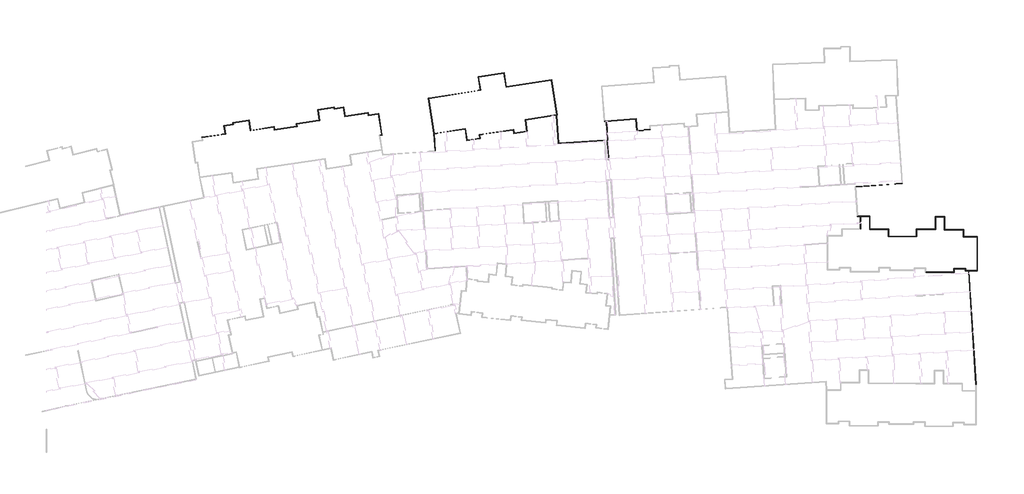
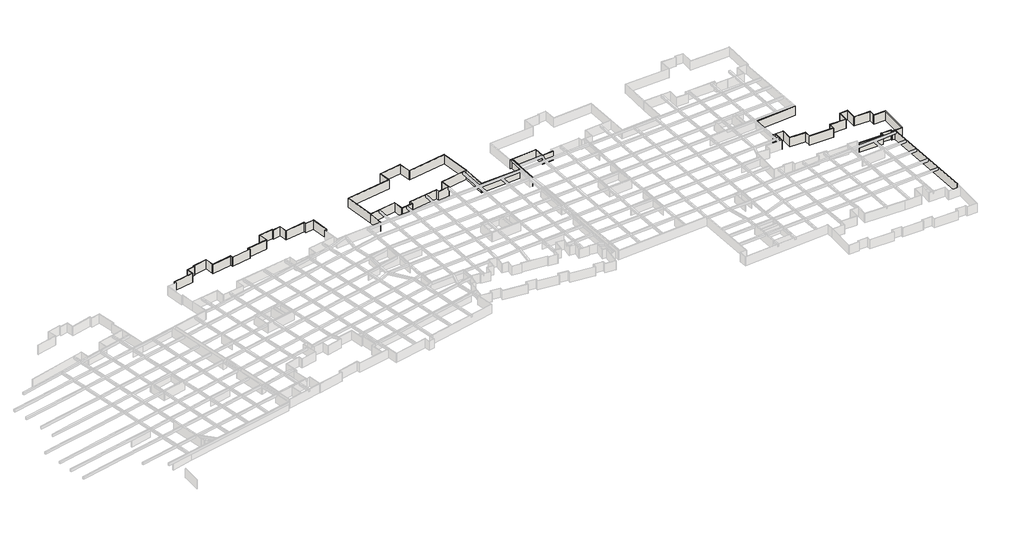
# One storey, part 6 of 14: 66 walls.
"""IFC4 building model written with IfcOpenShell, lengths in millimetres."""

from ifc_helpers import new_model, si_unit, origin, origin_with_axes, place, context, project, spatial, polyline, outline, extrude, faceted_brep, element, save

model = new_model("IFC4")

# Units and contexts
model_context = context("Model", 3, world=origin())
ifc_project = project(units=[si_unit("LENGTHUNIT", "METRE", prefix="MILLI")], contexts=[model_context])

# Site, building, storey
site = spatial("IfcSite", under=ifc_project)
building = spatial("IfcBuilding", under=site)
storey = spatial("IfcBuildingStorey", under=building, Name="户型图", Elevation=0.0)

# Walls
placement = place(None, origin())
element("IfcWall", 1, ObjectType="所有墙体", at=placement, inside=storey, context=model_context, shape_type="Brep", body=[
    faceted_brep([(-63852.357784, -149438.6682209, 0.0), (-63852.357784, -153118.7611434, 0.0), (-63852.357784, -153238.7611434, 0.0), (-63852.357784, -153238.7611434, 3300.0), (-63852.357784, -153118.7611434, 3300.0), (-63852.357784, -149438.6682209, 3300.0), (-63732.357784, -149438.6682209, 0.0), (-63732.357784, -149438.6682209, 3300.0), (-63732.357784, -153238.7611434, 3300.0), (-63732.357784, -153238.7611434, 0.0)], [[[0, 1, 2, 3, 4, 5]], [[6, 7, 8, 9]], [[2, 1, 0, 6, 9]], [[5, 4, 3, 8, 7]], [[3, 2, 9, 8]], [[0, 5, 7, 6]]]),
])
element("IfcWall", 2, ObjectType="所有墙体", at=placement, inside=storey, context=model_context, shape_type="Brep", body=[
    faceted_brep([(-44489.8483382, -166077.0504792, 0.0), (-36098.0374087, -166077.0504792, 0.0), (-36098.0374087, -166077.0504792, 3300.0), (-44489.8483382, -166077.0504792, 3300.0), (-44489.8483382, -165957.0504792, 0.0), (-44489.8483382, -165957.0504792, 3300.0), (-36218.0374087, -165957.0504792, 3300.0), (-36098.0374087, -165957.0504792, 3300.0), (-36098.0374087, -165957.0504792, 0.0), (-36218.0374087, -165957.0504792, 0.0)], [[[0, 1, 2, 3]], [[4, 5, 6, 7, 8, 9]], [[1, 0, 4, 9, 8]], [[3, 2, 7, 6, 5]], [[0, 3, 5, 4]], [[2, 1, 8, 7]]]),
])
element("IfcWall", 3, ObjectType="所有墙体", at=placement, inside=storey, context=model_context, shape_type="Brep", body=[
    faceted_brep([(-36098.0374087, -165957.0504792, 0.0), (-36098.0374087, -165032.3015604, 0.0), (-36098.0374087, -164912.3015604, 0.0), (-36098.0374087, -164817.0504792, 0.0), (-36098.0374087, -164817.0504792, 3300.0), (-36098.0374087, -164912.3015604, 3300.0), (-36098.0374087, -165032.3015604, 3300.0), (-36098.0374087, -165957.0504792, 3300.0), (-36218.0374087, -165957.0504792, 0.0), (-36218.0374087, -165957.0504792, 3300.0), (-36218.0374087, -164817.0504792, 3300.0), (-36218.0374087, -164817.0504792, 0.0)], [[[0, 1, 2, 3, 4, 5, 6, 7]], [[8, 9, 10, 11]], [[3, 2, 1, 0, 8, 11]], [[4, 3, 11, 10]], [[7, 6, 5, 4, 10, 9]], [[0, 7, 9, 8]]]),
])
element("IfcWall", 4, ObjectType="所有墙体", at=placement, inside=storey, context=model_context, shape_type="Brep", body=[
    faceted_brep([(-36098.0374087, -165032.3015604, 0.0), (-32810.647962, -165032.3015604, 0.0), (-32690.647962, -165032.3015604, 0.0), (-32690.647962, -165032.3015604, 3300.0), (-32810.647962, -165032.3015604, 3300.0), (-36098.0374087, -165032.3015604, 3300.0), (-36098.0374087, -164912.3015604, 0.0), (-36098.0374087, -164912.3015604, 3300.0), (-32690.647962, -164912.3015604, 3300.0), (-32690.647962, -164912.3015604, 0.0)], [[[0, 1, 2, 3, 4, 5]], [[6, 7, 8, 9]], [[2, 1, 0, 6, 9]], [[5, 4, 3, 8, 7]], [[0, 5, 7, 6]], [[3, 2, 9, 8]]]),
])
element("IfcWall", 5, ObjectType="所有墙体", at=placement, inside=storey, context=model_context, shape_type="Brep", body=[
    faceted_brep([(-32810.647962, -165032.3015604, 0.0), (-32810.647962, -165556.1428891, 0.0), (-32810.647962, -165556.1428891, 3300.0), (-32810.647962, -165032.3015604, 3300.0), (-32690.647962, -165032.3015604, 0.0), (-32690.647962, -165032.3015604, 3300.0), (-32690.647962, -165436.1428891, 3300.0), (-32690.647962, -165556.1428891, 3300.0), (-32690.647962, -165556.1428891, 0.0), (-32690.647962, -165436.1428891, 0.0)], [[[0, 1, 2, 3]], [[4, 5, 6, 7, 8, 9]], [[1, 0, 4, 9, 8]], [[3, 2, 7, 6, 5]], [[0, 3, 5, 4]], [[2, 1, 8, 7]]]),
])
element("IfcWall", 6, ObjectType="所有墙体", at=placement, inside=storey, context=model_context, shape_type="Brep", body=[
    faceted_brep([(-32690.647962, -165556.1428891, 0.0), (-31833.0771773, -165556.1428891, 0.0), (-31712.8241848, -165556.1428891, 0.0), (-29194.2257868, -165556.1428891, 0.0), (-29194.2257868, -165556.1428891, 3300.0), (-31712.8241848, -165556.1428891, 3300.0), (-31833.0771773, -165556.1428891, 3300.0), (-32690.647962, -165556.1428891, 3300.0), (-32690.647962, -165436.1428891, 0.0), (-32690.647962, -165436.1428891, 3300.0), (-29314.2257868, -165436.1428891, 3300.0), (-29194.2257868, -165436.1428891, 3300.0), (-29194.2257868, -165436.1428891, 0.0), (-29314.2257868, -165436.1428891, 0.0)], [[[0, 1, 2, 3, 4, 5, 6, 7]], [[8, 9, 10, 11, 12, 13]], [[3, 2, 1, 0, 8, 13, 12]], [[7, 6, 5, 4, 11, 10, 9]], [[0, 7, 9, 8]], [[4, 3, 12, 11]]]),
])
element("IfcWall", 7, ObjectType="所有墙体", at=placement, inside=storey, context=model_context, shape_type="Brep", body=[
    faceted_brep([(-29194.2257868, -165436.1428891, 0.0), (-29194.2257868, -155436.1428891, 0.0), (-29194.2257868, -155436.1428891, 3300.0), (-29194.2257868, -165436.1428891, 3300.0), (-29314.2257868, -165436.1428891, 0.0), (-29314.2257868, -165436.1428891, 3300.0), (-29314.2257868, -155556.1428891, 3300.0), (-29314.2257868, -155436.1428891, 3300.0), (-29314.2257868, -155436.1428891, 0.0), (-29314.2257868, -155556.1428891, 0.0)], [[[0, 1, 2, 3]], [[4, 5, 6, 7, 8, 9]], [[1, 0, 4, 9, 8]], [[3, 2, 7, 6, 5]], [[0, 3, 5, 4]], [[2, 1, 8, 7]]]),
])
element("IfcWall", 8, ObjectType="所有墙体", at=placement, inside=storey, context=model_context, shape_type="Brep", body=[
    faceted_brep([(-29314.2257868, -155436.1428891, 0.0), (-33294.2257868, -155436.1428891, 0.0), (-33414.2257868, -155436.1428891, 0.0), (-33414.2257868, -155436.1428891, 3300.0), (-33294.2257868, -155436.1428891, 3300.0), (-29314.2257868, -155436.1428891, 3300.0), (-29314.2257868, -155556.1428891, 0.0), (-29314.2257868, -155556.1428891, 3300.0), (-33414.2257868, -155556.1428891, 3300.0), (-33414.2257868, -155556.1428891, 0.0)], [[[0, 1, 2, 3, 4, 5]], [[6, 7, 8, 9]], [[2, 1, 0, 6, 9]], [[5, 4, 3, 8, 7]], [[0, 5, 7, 6]], [[3, 2, 9, 8]]]),
])
element("IfcWall", 9, ObjectType="所有墙体", at=placement, inside=storey, context=model_context, shape_type="Brep", body=[
    faceted_brep([(-33294.2257868, -155436.1428891, 0.0), (-33294.2257868, -153331.6259677, 0.0), (-33294.2257868, -153331.6259677, 3300.0), (-33294.2257868, -155436.1428891, 3300.0), (-33414.2257868, -155436.1428891, 0.0), (-33414.2257868, -155436.1428891, 3300.0), (-33414.2257868, -153451.6259677, 3300.0), (-33414.2257868, -153331.6259677, 3300.0), (-33414.2257868, -153331.6259677, 0.0), (-33414.2257868, -153451.6259677, 0.0)], [[[0, 1, 2, 3]], [[4, 5, 6, 7, 8, 9]], [[1, 0, 4, 9, 8]], [[3, 2, 7, 6, 5]], [[0, 3, 5, 4]], [[2, 1, 8, 7]]]),
])
element("IfcWall", 10, ObjectType="所有墙体", at=placement, inside=storey, context=model_context, shape_type="Brep", body=[
    faceted_brep([(-33414.2257868, -153331.6259677, 0.0), (-38859.8129577, -153331.6259677, 0.0), (-38979.8129577, -153331.6259677, 0.0), (-38979.8129577, -153331.6259677, 3300.0), (-38859.8129577, -153331.6259677, 3300.0), (-33414.2257868, -153331.6259677, 3300.0), (-33414.2257868, -153451.6259677, 0.0), (-33414.2257868, -153451.6259677, 3300.0), (-38979.8129577, -153451.6259677, 3300.0), (-38979.8129577, -153451.6259677, 0.0)], [[[0, 1, 2, 3, 4, 5]], [[6, 7, 8, 9]], [[2, 1, 0, 6, 9]], [[5, 4, 3, 8, 7]], [[0, 5, 7, 6]], [[3, 2, 9, 8]]]),
])
element("IfcWall", 11, ObjectType="所有墙体", at=placement, inside=storey, context=model_context, shape_type="Brep", body=[
    faceted_brep([(-38859.8129577, -153331.6259677, 0.0), (-38859.8129577, -149531.6259677, 0.0), (-38859.8129577, -149531.6259677, 3300.0), (-38859.8129577, -153331.6259677, 3300.0), (-38979.8129577, -153331.6259677, 0.0), (-38979.8129577, -153331.6259677, 3300.0), (-38979.8129577, -149651.6259677, 3300.0), (-38979.8129577, -149531.6259677, 3300.0), (-38979.8129577, -149531.6259677, 0.0), (-38979.8129577, -149651.6259677, 0.0)], [[[0, 1, 2, 3]], [[4, 5, 6, 7, 8, 9]], [[1, 0, 4, 9, 8]], [[3, 2, 7, 6, 5]], [[0, 3, 5, 4]], [[2, 1, 8, 7]]]),
])
element("IfcWall", 12, ObjectType="所有墙体", at=placement, inside=storey, context=model_context, shape_type="Brep", body=[
    faceted_brep([(-38979.8129577, -149531.6259677, 0.0), (-41679.8129577, -149531.6259677, 0.0), (-41679.8129577, -149531.6259677, 3300.0), (-38979.8129577, -149531.6259677, 3300.0), (-38979.8129577, -149651.6259677, 0.0), (-38979.8129577, -149651.6259677, 3300.0), (-41559.8129577, -149651.6259677, 3300.0), (-41679.8129577, -149651.6259677, 3300.0), (-41679.8129577, -149651.6259677, 0.0), (-41559.8129577, -149651.6259677, 0.0)], [[[0, 1, 2, 3]], [[4, 5, 6, 7, 8, 9]], [[1, 0, 4, 9, 8]], [[3, 2, 7, 6, 5]], [[0, 3, 5, 4]], [[2, 1, 8, 7]]]),
])
element("IfcWall", 13, ObjectType="所有墙体", at=placement, inside=storey, context=model_context, shape_type="Brep", body=[
    faceted_brep([(-41679.8129577, -149651.6259677, 0.0), (-41679.8129577, -153231.6259677, 0.0), (-41679.8129577, -153351.6259677, 0.0), (-41679.8129577, -153351.6259677, 3300.0), (-41679.8129577, -153231.6259677, 3300.0), (-41679.8129577, -149651.6259677, 3300.0), (-41559.8129577, -149651.6259677, 0.0), (-41559.8129577, -149651.6259677, 3300.0), (-41559.8129577, -153351.6259677, 3300.0), (-41559.8129577, -153351.6259677, 0.0)], [[[0, 1, 2, 3, 4, 5]], [[6, 7, 8, 9]], [[2, 1, 0, 6, 9]], [[5, 4, 3, 8, 7]], [[0, 5, 7, 6]], [[3, 2, 9, 8]]]),
])
element("IfcWall", 14, ObjectType="所有墙体", at=placement, inside=storey, context=model_context, shape_type="Brep", body=[
    faceted_brep([(-41679.8129577, -153231.6259677, 0.0), (-47279.8129577, -153231.6259677, 0.0), (-47279.8129577, -153231.6259677, 3300.0), (-41679.8129577, -153231.6259677, 3300.0), (-41679.8129577, -153351.6259677, 0.0), (-41679.8129577, -153351.6259677, 3300.0), (-47159.8129577, -153351.6259677, 3300.0), (-47279.8129577, -153351.6259677, 3300.0), (-47279.8129577, -153351.6259677, 0.0), (-47159.8129577, -153351.6259677, 0.0)], [[[0, 1, 2, 3]], [[4, 5, 6, 7, 8, 9]], [[1, 0, 4, 9, 8]], [[3, 2, 7, 6, 5]], [[0, 3, 5, 4]], [[2, 1, 8, 7]]]),
])
element("IfcWall", 15, ObjectType="所有墙体", at=placement, inside=storey, context=model_context, shape_type="Brep", body=[
    faceted_brep([(-47279.8129577, -153351.6259677, 0.0), (-47279.8129577, -155331.6259677, 0.0), (-47279.8129577, -155451.6259677, 0.0), (-47279.8129577, -155451.6259677, 3300.0), (-47279.8129577, -155331.6259677, 3300.0), (-47279.8129577, -153351.6259677, 3300.0), (-47159.8129577, -153351.6259677, 0.0), (-47159.8129577, -153351.6259677, 3300.0), (-47159.8129577, -155451.6259677, 3300.0), (-47159.8129577, -155451.6259677, 0.0)], [[[0, 1, 2, 3, 4, 5]], [[6, 7, 8, 9]], [[2, 1, 0, 6, 9]], [[5, 4, 3, 8, 7]], [[0, 5, 7, 6]], [[3, 2, 9, 8]]]),
])
element("IfcWall", 16, ObjectType="所有墙体", at=placement, inside=storey, context=model_context, shape_type="Brep", body=[
    faceted_brep([(-47279.8129577, -155331.6259677, 0.0), (-55524.2068249, -155331.6259677, 0.0), (-55644.2068249, -155331.6259677, 0.0), (-55644.2068249, -155331.6259677, 3300.0), (-55524.2068249, -155331.6259677, 3300.0), (-47279.8129577, -155331.6259677, 3300.0), (-47279.8129577, -155451.6259677, 0.0), (-47279.8129577, -155451.6259677, 3300.0), (-55644.2068249, -155451.6259677, 3300.0), (-55644.2068249, -155451.6259677, 0.0)], [[[0, 1, 2, 3, 4, 5]], [[6, 7, 8, 9]], [[2, 1, 0, 6, 9]], [[5, 4, 3, 8, 7]], [[0, 5, 7, 6]], [[3, 2, 9, 8]]]),
])
element("IfcWall", 17, ObjectType="所有墙体", at=placement, inside=storey, context=model_context, shape_type="Brep", body=[
    faceted_brep([(-55524.2068249, -155331.6259677, 0.0), (-55524.2068249, -153151.6259677, 0.0), (-55524.2068249, -153151.6259677, 3300.0), (-55524.2068249, -155331.6259677, 3300.0), (-55644.2068249, -155331.6259677, 0.0), (-55644.2068249, -155331.6259677, 3300.0), (-55644.2068249, -153271.6259677, 3300.0), (-55644.2068249, -153151.6259677, 3300.0), (-55644.2068249, -153151.6259677, 0.0), (-55644.2068249, -153271.6259677, 0.0)], [[[0, 1, 2, 3]], [[4, 5, 6, 7, 8, 9]], [[1, 0, 4, 9, 8]], [[3, 2, 7, 6, 5]], [[0, 3, 5, 4]], [[2, 1, 8, 7]]]),
])
element("IfcWall", 18, ObjectType="所有墙体", at=placement, inside=storey, context=model_context, shape_type="Brep", body=[
    faceted_brep([(-55644.2068249, -153151.6259677, 0.0), (-61024.2068249, -153151.6259677, 0.0), (-61144.2068249, -153151.6259677, 0.0), (-61144.2068249, -153151.6259677, 3300.0), (-61024.2068249, -153151.6259677, 3300.0), (-55644.2068249, -153151.6259677, 3300.0), (-55644.2068249, -153271.6259677, 0.0), (-55644.2068249, -153271.6259677, 3300.0), (-61144.2068249, -153271.6259677, 3300.0), (-61144.2068249, -153271.6259677, 0.0)], [[[0, 1, 2, 3, 4, 5]], [[6, 7, 8, 9]], [[2, 1, 0, 6, 9]], [[5, 4, 3, 8, 7]], [[0, 5, 7, 6]], [[3, 2, 9, 8]]]),
])
element("IfcWall", 19, ObjectType="所有墙体", at=placement, inside=storey, context=model_context, shape_type="Brep", body=[
    faceted_brep([(-61024.2068249, -153151.6259677, 0.0), (-61024.2068249, -149318.6682209, 0.0), (-61024.2068249, -149318.6682209, 3300.0), (-61024.2068249, -153151.6259677, 3300.0), (-61144.2068249, -153151.6259677, 0.0), (-61144.2068249, -153151.6259677, 3300.0), (-61144.2068249, -149438.6682209, 3300.0), (-61144.2068249, -149318.6682209, 3300.0), (-61144.2068249, -149318.6682209, 0.0), (-61144.2068249, -149438.6682209, 0.0)], [[[0, 1, 2, 3]], [[4, 5, 6, 7, 8, 9]], [[1, 0, 4, 9, 8]], [[3, 2, 7, 6, 5]], [[0, 3, 5, 4]], [[2, 1, 8, 7]]]),
])
element("IfcWall", 20, ObjectType="所有墙体", at=placement, inside=storey, context=model_context, shape_type="Brep", body=[
    faceted_brep([(-61144.2068249, -149318.6682209, 0.0), (-64662.1102247, -149318.6682209, 0.0), (-64782.4032525, -149318.6682209, 0.0), (-64782.4032525, -149318.6682209, 3300.0), (-64662.1102247, -149318.6682209, 3300.0), (-61144.2068249, -149318.6682209, 3300.0), (-61144.2068249, -149438.6682209, 0.0), (-61144.2068249, -149438.6682209, 3300.0), (-63732.357784, -149438.6682209, 3300.0), (-63852.357784, -149438.6682209, 3300.0), (-64774.0120351, -149438.6682209, 3300.0), (-64774.0120351, -149438.6682209, 0.0), (-63852.357784, -149438.6682209, 0.0), (-63732.357784, -149438.6682209, 0.0)], [[[0, 1, 2, 3, 4, 5]], [[6, 7, 8, 9, 10, 11, 12, 13]], [[2, 1, 0, 6, 13, 12, 11]], [[5, 4, 3, 10, 9, 8, 7]], [[0, 5, 7, 6]], [[3, 2, 11, 10]]]),
])
element("IfcWall", 21, ObjectType="所有墙体", at=placement, inside=storey, context=model_context, shape_type="Brep", body=[
    faceted_brep([(-139619.0065176, -121289.1155096, 0.0), (-139081.9141821, -121248.6544174, 0.0), (-138962.222053, -121239.63758, 0.0), (-130362.6959186, -120591.8044292, 0.0), (-130243.034985, -120582.7899419, 0.0), (-130243.034985, -120582.7899419, 3300.0), (-130362.6959186, -120591.8044292, 3300.0), (-138962.222053, -121239.63758, 3300.0), (-139081.9141821, -121248.6544174, 3300.0), (-139619.0065176, -121289.1155096, 3300.0), (-139628.021005, -121169.4545761, 0.0), (-139628.021005, -121169.4545761, 3300.0), (-130252.0494724, -120463.1290083, 3300.0), (-130252.0494724, -120463.1290083, 0.0)], [[[0, 1, 2, 3, 4, 5, 6, 7, 8, 9]], [[10, 11, 12, 13]], [[4, 3, 2, 1, 0, 10, 13]], [[9, 8, 7, 6, 5, 12, 11]], [[0, 9, 11, 10]], [[5, 4, 13, 12]]]),
])
element("IfcWall", 22, ObjectType="所有墙体", at=placement, inside=storey, context=model_context, shape_type="Brep", body=[
    faceted_brep([(-130362.6959186, -120591.8044292, 0.0), (-130099.9459312, -124079.6243728, 0.0), (-130099.9459312, -124079.6243728, 3300.0), (-130362.6959186, -120591.8044292, 3300.0), (-130243.034985, -120582.7899419, 0.0), (-130243.034985, -120582.7899419, 3300.0), (-129989.299485, -123950.9489519, 3300.0), (-129980.2849976, -124070.6098855, 3300.0), (-129980.2849976, -124070.6098855, 0.0), (-129989.299485, -123950.9489519, 0.0)], [[[0, 1, 2, 3]], [[4, 5, 6, 7, 8, 9]], [[1, 0, 4, 9, 8]], [[3, 2, 7, 6, 5]], [[0, 3, 5, 4]], [[2, 1, 8, 7]]]),
])
element("IfcWall", 23, ObjectType="所有墙体", at=placement, inside=storey, context=model_context, shape_type="Brep", body=[
    faceted_brep([(-129980.2849976, -124070.6098855, 0.0), (-126090.4525069, -123777.5748509, 0.0), (-126090.4525069, -123777.5748509, 3300.0), (-129980.2849976, -124070.6098855, 3300.0), (-129989.299485, -123950.9489519, 0.0), (-129989.299485, -123950.9489519, 3300.0), (-126219.1279278, -123666.9284047, 3300.0), (-126099.4669943, -123657.9139173, 3300.0), (-126099.4669943, -123657.9139173, 0.0), (-126219.1279278, -123666.9284047, 0.0)], [[[0, 1, 2, 3]], [[4, 5, 6, 7, 8, 9]], [[1, 0, 4, 9, 8]], [[3, 2, 7, 6, 5]], [[0, 3, 5, 4]], [[2, 1, 8, 7]]]),
])
element("IfcWall", 24, ObjectType="所有墙体", at=placement, inside=storey, context=model_context, shape_type="Brep", body=[
    faceted_brep([(-190088.7056475, -124948.17441, 0.0), (-190107.4777833, -124829.6518091, 0.0), (-191744.4589692, -114494.1593671, 0.0), (-191763.231105, -114375.6367662, 0.0), (-191763.231105, -114375.6367662, 3300.0), (-191744.4589692, -114494.1593671, 3300.0), (-190107.4777833, -124829.6518091, 3300.0), (-190088.7056475, -124948.17441, 3300.0), (-190207.2282484, -124966.9465458, 0.0), (-190207.2282484, -124966.9465458, 3300.0), (-191881.7537059, -114394.408902, 3300.0), (-191881.7537059, -114394.408902, 0.0), (-190093.6639709, -124948.9597313, 0.0), (-190093.6639709, -124948.9597313, 3300.0)], [[[0, 1, 2, 3, 4, 5, 6, 7]], [[8, 9, 10, 11]], [[3, 2, 1, 0, 12, 8, 11]], [[7, 6, 5, 4, 10, 9, 13]], [[4, 3, 11, 10]], [[0, 7, 13, 9, 8, 12]]]),
])
element("IfcWall", 25, ObjectType="所有墙体", at=placement, inside=storey, context=model_context, shape_type="Brep", body=[
    faceted_brep([(-191744.4589692, -114494.1593671, 0.0), (-176350.1815066, -112055.945347, 0.0), (-176350.1815066, -112055.945347, 3300.0), (-191744.4589692, -114494.1593671, 3300.0), (-191763.231105, -114375.6367662, 0.0), (-191763.231105, -114375.6367662, 3300.0), (-176487.4762433, -111956.1948819, 3300.0), (-176368.9536424, -111937.4227461, 3300.0), (-176368.9536424, -111937.4227461, 0.0), (-176487.4762433, -111956.1948819, 0.0)], [[[0, 1, 2, 3]], [[4, 5, 6, 7, 8, 9]], [[1, 0, 4, 9, 8]], [[3, 2, 7, 6, 5]], [[0, 3, 5, 4]], [[2, 1, 8, 7]]]),
])
element("IfcWall", 26, ObjectType="所有墙体", at=placement, inside=storey, context=model_context, shape_type="Brep", body=[
    faceted_brep([(-176368.9536424, -111937.4227461, 0.0), (-176969.7169507, -108144.3524984, 0.0), (-176988.4890865, -108025.8298976, 0.0), (-176988.4890865, -108025.8298976, 3300.0), (-176969.7169507, -108144.3524984, 3300.0), (-176368.9536424, -111937.4227461, 3300.0), (-176487.4762433, -111956.1948819, 0.0), (-176487.4762433, -111956.1948819, 3300.0), (-177107.0116874, -108044.6020334, 3300.0), (-177107.0116874, -108044.6020334, 0.0)], [[[0, 1, 2, 3, 4, 5]], [[6, 7, 8, 9]], [[2, 1, 0, 6, 9]], [[5, 4, 3, 8, 7]], [[0, 5, 7, 6]], [[3, 2, 9, 8]]]),
])
element("IfcWall", 27, ObjectType="所有墙体", at=placement, inside=storey, context=model_context, shape_type="Brep", body=[
    faceted_brep([(-176969.7169507, -108144.3524984, 0.0), (-169496.9225676, -106960.7781424, 0.0), (-169378.3999667, -106942.0060066, 0.0), (-169378.3999667, -106942.0060066, 3300.0), (-169496.9225676, -106960.7781424, 3300.0), (-176969.7169507, -108144.3524984, 3300.0), (-176988.4890865, -108025.8298976, 0.0), (-176988.4890865, -108025.8298976, 3300.0), (-169397.1721025, -106823.4834057, 3300.0), (-169397.1721025, -106823.4834057, 0.0)], [[[0, 1, 2, 3, 4, 5]], [[6, 7, 8, 9]], [[2, 1, 0, 6, 9]], [[5, 4, 3, 8, 7]], [[0, 5, 7, 6]], [[3, 2, 9, 8]]]),
])
element("IfcWall", 28, ObjectType="所有墙体", at=placement, inside=storey, context=model_context, shape_type="Brep", body=[
    faceted_brep([(-169496.9225676, -106960.7781424, 0.0), (-168829.0528733, -111177.5414362, 0.0), (-168829.0528733, -111177.5414362, 3300.0), (-169496.9225676, -106960.7781424, 3300.0), (-169378.3999667, -106942.0060066, 0.0), (-169378.3999667, -106942.0060066, 3300.0), (-168729.3024082, -111040.2466995, 3300.0), (-168710.5302724, -111158.7693004, 3300.0), (-168710.5302724, -111158.7693004, 0.0), (-168729.3024082, -111040.2466995, 0.0)], [[[0, 1, 2, 3]], [[4, 5, 6, 7, 8, 9]], [[1, 0, 4, 9, 8]], [[3, 2, 7, 6, 5]], [[0, 3, 5, 4]], [[2, 1, 8, 7]]]),
])
element("IfcWall", 29, ObjectType="所有墙体", at=placement, inside=storey, context=model_context, shape_type="Brep", body=[
    faceted_brep([(-168710.5302724, -111158.7693004, 0.0), (-155433.8901305, -109055.9560821, 0.0), (-155315.3675296, -109037.1839463, 0.0), (-155315.3675296, -109037.1839463, 3300.0), (-155433.8901305, -109055.9560821, 3300.0), (-168710.5302724, -111158.7693004, 3300.0), (-168729.3024082, -111040.2466995, 0.0), (-168729.3024082, -111040.2466995, 3300.0), (-155334.1396655, -108918.6613454, 3300.0), (-155334.1396655, -108918.6613454, 0.0)], [[[0, 1, 2, 3, 4, 5]], [[6, 7, 8, 9]], [[2, 1, 0, 6, 9]], [[5, 4, 3, 8, 7]], [[0, 5, 7, 6]], [[3, 2, 9, 8]]]),
])
element("IfcWall", 30, ObjectType="所有墙体", at=placement, inside=storey, context=model_context, shape_type="Brep", body=[
    faceted_brep([(-155433.8901305, -109055.9560821, 0.0), (-153806.588586, -119330.3336735, 0.0), (-153787.8164502, -119448.8562744, 0.0), (-153787.8164502, -119448.8562744, 3300.0), (-153806.588586, -119330.3336735, 3300.0), (-155433.8901305, -109055.9560821, 3300.0), (-155315.3675296, -109037.1839463, 0.0), (-155315.3675296, -109037.1839463, 3300.0), (-153669.2938493, -119430.0841386, 3300.0), (-153669.2938493, -119430.0841386, 0.0)], [[[0, 1, 2, 3, 4, 5]], [[6, 7, 8, 9]], [[2, 1, 0, 6, 9]], [[5, 4, 3, 8, 7]], [[0, 5, 7, 6]], [[3, 2, 9, 8]]]),
])
element("IfcWall", 31, ObjectType="所有墙体", at=placement, inside=storey, context=model_context, shape_type="Brep", body=[
    faceted_brep([(-153806.588586, -119330.3336735, 0.0), (-163184.7449291, -120815.6877172, 0.0), (-163184.7449291, -120815.6877172, 3300.0), (-153806.588586, -119330.3336735, 3300.0), (-153787.8164502, -119448.8562744, 0.0), (-153787.8164502, -119448.8562744, 3300.0), (-153799.2876915, -119450.6731405, 3300.0), (-153918.3434665, -119469.5297228, 3300.0), (-163047.4501924, -120915.4381823, 3300.0), (-163165.9727933, -120934.2103181, 3300.0), (-163165.9727933, -120934.2103181, 0.0), (-163047.4501924, -120915.4381823, 0.0), (-153918.3434665, -119469.5297228, 0.0), (-153799.2876915, -119450.6731405, 0.0)], [[[0, 1, 2, 3]], [[4, 5, 6, 7, 8, 9, 10, 11, 12, 13]], [[1, 0, 4, 13, 12, 11, 10]], [[3, 2, 9, 8, 7, 6, 5]], [[0, 3, 5, 4]], [[2, 1, 10, 9]]]),
])
element("IfcWall", 32, ObjectType="所有墙体", at=placement, inside=storey, context=model_context, shape_type="Brep", body=[
    faceted_brep([(-163165.9727933, -120934.2103181, 0.0), (-162650.5667245, -124188.3561656, 0.0), (-162631.7945887, -124306.8787665, 0.0), (-162631.7945887, -124306.8787665, 3300.0), (-162650.5667245, -124188.3561656, 3300.0), (-163165.9727933, -120934.2103181, 3300.0), (-163047.4501924, -120915.4381823, 0.0), (-163047.4501924, -120915.4381823, 3300.0), (-162513.2719878, -124288.1066307, 3300.0), (-162513.2719878, -124288.1066307, 0.0)], [[[0, 1, 2, 3, 4, 5]], [[6, 7, 8, 9]], [[2, 1, 0, 6, 9]], [[5, 4, 3, 8, 7]], [[0, 5, 7, 6]], [[3, 2, 9, 8]]]),
])
element("IfcWall", 33, ObjectType="所有墙体", at=placement, inside=storey, context=model_context, shape_type="Brep", body=[
    faceted_brep([(-162650.5667245, -124188.3561656, 0.0), (-166414.5336953, -124784.5099677, 0.0), (-166533.0562961, -124803.2821035, 0.0), (-166533.0562961, -124803.2821035, 3300.0), (-166414.5336953, -124784.5099677, 3300.0), (-162650.5667245, -124188.3561656, 3300.0), (-162631.7945887, -124306.8787665, 0.0), (-162631.7945887, -124306.8787665, 3300.0), (-166514.2841603, -124921.8047043, 3300.0), (-166514.2841603, -124921.8047043, 0.0)], [[[0, 1, 2, 3, 4, 5]], [[6, 7, 8, 9]], [[2, 1, 0, 6, 9]], [[5, 4, 3, 8, 7]], [[0, 5, 7, 6]], [[3, 2, 9, 8]]]),
])
element("IfcWall", 34, ObjectType="所有墙体", at=placement, inside=storey, context=model_context, shape_type="Brep", body=[
    faceted_brep([(-166414.5336953, -124784.5099677, 0.0), (-166586.4492021, -123699.0781757, 0.0), (-166586.4492021, -123699.0781757, 3300.0), (-166414.5336953, -124784.5099677, 3300.0), (-166533.0562961, -124803.2821035, 0.0), (-166533.0562961, -124803.2821035, 3300.0), (-166686.5244765, -123834.322147, 3300.0), (-166705.2994719, -123715.7814918, 3300.0), (-166705.2994719, -123715.7814918, 0.0), (-166686.5244765, -123834.322147, 0.0)], [[[0, 1, 2, 3]], [[4, 5, 6, 7, 8, 9]], [[1, 0, 4, 9, 8]], [[3, 2, 7, 6, 5]], [[0, 3, 5, 4]], [[2, 1, 8, 7]]]),
])
element("IfcWall", 35, ObjectType="所有墙体", at=placement, inside=storey, context=model_context, shape_type="Brep", body=[
    faceted_brep([(-166705.2994719, -123715.7814918, 0.0), (-176806.033773, -125135.3471216, 0.0), (-176806.033773, -125135.3471216, 3300.0), (-166705.2994719, -123715.7814918, 3300.0), (-166686.5244765, -123834.322147, 0.0), (-166686.5244765, -123834.322147, 3300.0), (-176668.408508, -125237.1844607, 3300.0), (-176787.2587777, -125253.8877768, 3300.0), (-176787.2587777, -125253.8877768, 0.0), (-176668.408508, -125237.1844607, 0.0)], [[[0, 1, 2, 3]], [[4, 5, 6, 7, 8, 9]], [[1, 0, 4, 9, 8]], [[3, 2, 7, 6, 5]], [[0, 3, 5, 4]], [[2, 1, 8, 7]]]),
])
element("IfcWall", 36, ObjectType="所有墙体", at=placement, inside=storey, context=model_context, shape_type="Brep", body=[
    faceted_brep([(-176787.2587777, -125253.8877768, 0.0), (-176618.312415, -126320.5731303, 0.0), (-176599.5374196, -126439.1137855, 0.0), (-176599.5374196, -126439.1137855, 3300.0), (-176618.312415, -126320.5731303, 3300.0), (-176787.2587777, -125253.8877768, 3300.0), (-176668.408508, -125237.1844607, 0.0), (-176668.408508, -125237.1844607, 3300.0), (-176480.6871499, -126422.4104694, 3300.0), (-176480.6871499, -126422.4104694, 0.0)], [[[0, 1, 2, 3, 4, 5]], [[6, 7, 8, 9]], [[2, 1, 0, 6, 9]], [[5, 4, 3, 8, 7]], [[0, 5, 7, 6]], [[3, 2, 9, 8]]]),
])
element("IfcWall", 37, ObjectType="所有墙体", at=placement, inside=storey, context=model_context, shape_type="Brep", body=[
    faceted_brep([(-176618.312415, -126320.5731303, 0.0), (-180360.4795525, -126846.5004234, 0.0), (-180479.3117207, -126863.2011955, 0.0), (-180479.3117207, -126863.2011955, 3300.0), (-180360.4795525, -126846.5004234, 3300.0), (-176618.312415, -126320.5731303, 3300.0), (-176599.5374196, -126439.1137855, 0.0), (-176599.5374196, -126439.1137855, 3300.0), (-180462.6109486, -126982.0333638, 3300.0), (-180462.6109486, -126982.0333638, 0.0)], [[[0, 1, 2, 3, 4, 5]], [[6, 7, 8, 9]], [[2, 1, 0, 6, 9]], [[5, 4, 3, 8, 7]], [[0, 5, 7, 6]], [[3, 2, 9, 8]]]),
])
element("IfcWall", 38, ObjectType="所有墙体", at=placement, inside=storey, context=model_context, shape_type="Brep", body=[
    faceted_brep([(-180360.4795525, -126846.5004234, 0.0), (-180849.9958867, -123363.4107201, 0.0), (-180849.9958867, -123363.4107201, 3300.0), (-180360.4795525, -126846.5004234, 3300.0), (-180479.3117207, -126863.2011955, 0.0), (-180479.3117207, -126863.2011955, 3300.0), (-180951.8332258, -123501.0359852, 3300.0), (-180968.5365419, -123382.1857155, 3300.0), (-180968.5365419, -123382.1857155, 0.0), (-180951.8332258, -123501.0359852, 0.0)], [[[0, 1, 2, 3]], [[4, 5, 6, 7, 8, 9]], [[1, 0, 4, 9, 8]], [[3, 2, 7, 6, 5]], [[0, 3, 5, 4]], [[2, 1, 8, 7]]]),
])
element("IfcWall", 39, ObjectType="所有墙体", at=placement, inside=storey, context=model_context, shape_type="SweptSolid", body=[
    extrude(outline(polyline([(-190107.4777833, -124829.6518091), (-180968.5365419, -123382.1857155), (-180951.8332258, -123501.0359852), (-190088.7056475, -124948.17441), (-190107.4777833, -124829.6518091)])), origin_with_axes(), (0.0, 0.0, 1.0), 3300.0),
])
element("IfcWall", 40, ObjectType="所有墙体", at=placement, inside=storey, context=model_context, shape_type="Brep", body=[
    faceted_brep([(-206189.3856367, -125435.3862189, 0.0), (-205557.5200855, -125335.3085472, 0.0), (-205557.5200855, -125335.3085472, 3300.0), (-206189.3856367, -125435.3862189, 3300.0), (-206208.1577725, -125316.863618, 0.0), (-206208.1577725, -125316.863618, 3300.0), (-205694.8148222, -125235.5580821, 3300.0), (-205576.2922213, -125216.7859463, 3300.0), (-205576.2922213, -125216.7859463, 0.0), (-205694.8148222, -125235.5580821, 0.0)], [[[0, 1, 2, 3]], [[4, 5, 6, 7, 8, 9]], [[1, 0, 4, 9, 8]], [[3, 2, 7, 6, 5]], [[0, 3, 5, 4]], [[2, 1, 8, 7]]]),
])
element("IfcWall", 41, ObjectType="所有墙体", at=placement, inside=storey, context=model_context, shape_type="Brep", body=[
    faceted_brep([(-205576.2922213, -125216.7859463, 0.0), (-206561.0118402, -118999.5109611, 0.0), (-206561.0118402, -118999.5109611, 3300.0), (-205576.2922213, -125216.7859463, 3300.0), (-205694.8148222, -125235.5580821, 0.0), (-205694.8148222, -125235.5580821, 3300.0), (-206660.7623052, -119136.8056977, 3300.0), (-206679.5344411, -119018.2830969, 3300.0), (-206679.5344411, -119018.2830969, 0.0), (-206660.7623052, -119136.8056977, 0.0)], [[[0, 1, 2, 3]], [[4, 5, 6, 7, 8, 9]], [[1, 0, 4, 9, 8]], [[3, 2, 7, 6, 5]], [[0, 3, 5, 4]], [[2, 1, 8, 7]]]),
])
element("IfcWall", 42, ObjectType="所有墙体", at=placement, inside=storey, context=model_context, shape_type="Brep", body=[
    faceted_brep([(-206679.5344411, -119018.2830969, 0.0), (-209469.3165861, -119460.1411805, 0.0), (-209587.839187, -119478.9133163, 0.0), (-209587.839187, -119478.9133163, 3300.0), (-209469.3165861, -119460.1411805, 3300.0), (-206679.5344411, -119018.2830969, 3300.0), (-206660.7623052, -119136.8056977, 0.0), (-206660.7623052, -119136.8056977, 3300.0), (-209569.0670512, -119597.4359172, 3300.0), (-209569.0670512, -119597.4359172, 0.0)], [[[0, 1, 2, 3, 4, 5]], [[6, 7, 8, 9]], [[2, 1, 0, 6, 9]], [[5, 4, 3, 8, 7]], [[0, 5, 7, 6]], [[3, 2, 9, 8]]]),
])
element("IfcWall", 43, ObjectType="所有墙体", at=placement, inside=storey, context=model_context, shape_type="Brep", body=[
    faceted_brep([(-209469.3165861, -119460.1411805, 0.0), (-209598.5347056, -118644.2900831, 0.0), (-209598.5347056, -118644.2900831, 3300.0), (-209469.3165861, -119460.1411805, 3300.0), (-209587.839187, -119478.9133163, 0.0), (-209587.839187, -119478.9133163, 3300.0), (-209698.2851706, -118781.5848198, 3300.0), (-209717.0573064, -118663.0622189, 3300.0), (-209717.0573064, -118663.0622189, 0.0), (-209698.2851706, -118781.5848198, 0.0)], [[[0, 1, 2, 3]], [[4, 5, 6, 7, 8, 9]], [[1, 0, 4, 9, 8]], [[3, 2, 7, 6, 5]], [[0, 3, 5, 4]], [[2, 1, 8, 7]]]),
])
element("IfcWall", 44, ObjectType="所有墙体", at=placement, inside=storey, context=model_context, shape_type="Brep", body=[
    faceted_brep([(-209717.0573064, -118663.0622189, 0.0), (-216505.4214218, -119738.2334701, 0.0), (-216623.9440227, -119757.0056059, 0.0), (-216623.9440227, -119757.0056059, 3300.0), (-216505.4214218, -119738.2334701, 3300.0), (-209717.0573064, -118663.0622189, 3300.0), (-209698.2851706, -118781.5848198, 0.0), (-209698.2851706, -118781.5848198, 3300.0), (-216605.1718869, -119875.5282067, 3300.0), (-216605.1718869, -119875.5282067, 0.0)], [[[0, 1, 2, 3, 4, 5]], [[6, 7, 8, 9]], [[2, 1, 0, 6, 9]], [[5, 4, 3, 8, 7]], [[0, 5, 7, 6]], [[3, 2, 9, 8]]]),
])
element("IfcWall", 45, ObjectType="所有墙体", at=placement, inside=storey, context=model_context, shape_type="Brep", body=[
    faceted_brep([(-216505.4214218, -119738.2334701, 0.0), (-216937.4664308, -117010.4086401, 0.0), (-216937.4664308, -117010.4086401, 3300.0), (-216505.4214218, -119738.2334701, 3300.0), (-216623.9440227, -119757.0056059, 0.0), (-216623.9440227, -119757.0056059, 3300.0), (-217037.2168959, -117147.7033768, 3300.0), (-217055.9890317, -117029.1807759, 3300.0), (-217055.9890317, -117029.1807759, 0.0), (-217037.2168959, -117147.7033768, 0.0)], [[[0, 1, 2, 3]], [[4, 5, 6, 7, 8, 9]], [[1, 0, 4, 9, 8]], [[3, 2, 7, 6, 5]], [[0, 3, 5, 4]], [[2, 1, 8, 7]]]),
])
element("IfcWall", 46, ObjectType="所有墙体", at=placement, inside=storey, context=model_context, shape_type="Brep", body=[
    faceted_brep([(-217055.9890317, -117029.1807759, 0.0), (-219604.2249504, -117432.7816957, 0.0), (-219722.7475513, -117451.5538315, 0.0), (-219722.7475513, -117451.5538315, 3300.0), (-219604.2249504, -117432.7816957, 3300.0), (-217055.9890317, -117029.1807759, 3300.0), (-217037.2168959, -117147.7033768, 0.0), (-217037.2168959, -117147.7033768, 3300.0), (-219703.9754155, -117570.0764324, 3300.0), (-219703.9754155, -117570.0764324, 0.0)], [[[0, 1, 2, 3, 4, 5]], [[6, 7, 8, 9]], [[2, 1, 0, 6, 9]], [[5, 4, 3, 8, 7]], [[0, 5, 7, 6]], [[3, 2, 9, 8]]]),
])
element("IfcWall", 47, ObjectType="所有墙体", at=placement, inside=storey, context=model_context, shape_type="Brep", body=[
    faceted_brep([(-219604.2249504, -117432.7816957, 0.0), (-219670.5291756, -117014.1532938, 0.0), (-219670.5291756, -117014.1532938, 3300.0), (-219604.2249504, -117432.7816957, 3300.0), (-219722.7475513, -117451.5538315, 0.0), (-219722.7475513, -117451.5538315, 3300.0), (-219770.2796406, -117151.4480305, 3300.0), (-219789.0517764, -117032.9254296, 3300.0), (-219789.0517764, -117032.9254296, 0.0), (-219770.2796406, -117151.4480305, 0.0)], [[[0, 1, 2, 3]], [[4, 5, 6, 7, 8, 9]], [[1, 0, 4, 9, 8]], [[3, 2, 7, 6, 5]], [[0, 3, 5, 4]], [[2, 1, 8, 7]]]),
])
element("IfcWall", 48, ObjectType="所有墙体", at=placement, inside=storey, context=model_context, shape_type="Brep", body=[
    faceted_brep([(-219789.0517764, -117032.9254296, 0.0), (-224628.7246453, -117799.4543083, 0.0), (-224628.7246453, -117799.4543083, 3300.0), (-219789.0517764, -117032.9254296, 3300.0), (-219770.2796406, -117151.4480305, 0.0), (-219770.2796406, -117151.4480305, 3300.0), (-224491.4299087, -117899.2047734, 3300.0), (-224609.9525095, -117917.9769092, 3300.0), (-224609.9525095, -117917.9769092, 0.0), (-224491.4299087, -117899.2047734, 0.0)], [[[0, 1, 2, 3]], [[4, 5, 6, 7, 8, 9]], [[1, 0, 4, 9, 8]], [[3, 2, 7, 6, 5]], [[0, 3, 5, 4]], [[2, 1, 8, 7]]]),
])
element("IfcWall", 49, ObjectType="所有墙体", at=placement, inside=storey, context=model_context, shape_type="Brep", body=[
    faceted_brep([(-224609.9525095, -117917.9769092, 0.0), (-224130.5406754, -120944.8641032, 0.0), (-224111.7656801, -121063.4047584, 0.0), (-224111.7656801, -121063.4047584, 3300.0), (-224130.5406754, -120944.8641032, 3300.0), (-224609.9525095, -117917.9769092, 3300.0), (-224491.4299087, -117899.2047734, 0.0), (-224491.4299087, -117899.2047734, 3300.0), (-223992.9154103, -121046.7014422, 3300.0), (-223992.9154103, -121046.7014422, 0.0)], [[[0, 1, 2, 3, 4, 5]], [[6, 7, 8, 9]], [[2, 1, 0, 6, 9]], [[5, 4, 3, 8, 7]], [[0, 5, 7, 6]], [[3, 2, 9, 8]]]),
])
element("IfcWall", 50, ObjectType="所有墙体", at=placement, inside=storey, context=model_context, shape_type="Brep", body=[
    faceted_brep([(-224130.5406754, -120944.8641032, 0.0), (-230963.3903497, -121905.1584998, 0.0), (-230963.3903497, -121905.1584998, 3300.0), (-224130.5406754, -120944.8641032, 3300.0), (-224111.7656801, -121063.4047584, 0.0), (-224111.7656801, -121063.4047584, 3300.0), (-230825.7650847, -122006.9958389, 3300.0), (-230944.6153544, -122023.699155, 3300.0), (-230944.6153544, -122023.699155, 0.0), (-230825.7650847, -122006.9958389, 0.0)], [[[0, 1, 2, 3]], [[4, 5, 6, 7, 8, 9]], [[1, 0, 4, 9, 8]], [[3, 2, 7, 6, 5]], [[0, 3, 5, 4]], [[2, 1, 8, 7]]]),
])
element("IfcWall", 51, ObjectType="所有墙体", at=placement, inside=storey, context=model_context, shape_type="Brep", body=[
    faceted_brep([(-230944.6153544, -122023.699155, 0.0), (-230838.0775135, -122696.3526093, 0.0), (-230819.3053777, -122814.8752101, 0.0), (-230819.3053777, -122814.8752101, 3300.0), (-230838.0775135, -122696.3526093, 3300.0), (-230944.6153544, -122023.699155, 3300.0), (-230825.7650847, -122006.9958389, 0.0), (-230825.7650847, -122006.9958389, 3300.0), (-230700.7827768, -122796.1030743, 3300.0), (-230700.7827768, -122796.1030743, 0.0)], [[[0, 1, 2, 3, 4, 5]], [[6, 7, 8, 9]], [[2, 1, 0, 6, 9]], [[5, 4, 3, 8, 7]], [[0, 5, 7, 6]], [[3, 2, 9, 8]]]),
])
element("IfcWall", 52, ObjectType="所有墙体", at=placement, inside=storey, context=model_context, shape_type="Brep", body=[
    faceted_brep([(-230838.0775135, -122696.3526093, 0.0), (-237344.8447036, -123726.923289, 0.0), (-237463.3673045, -123745.6954248, 0.0), (-237463.3673045, -123745.6954248, 3300.0), (-237344.8447036, -123726.923289, 3300.0), (-230838.0775135, -122696.3526093, 3300.0), (-230819.3053777, -122814.8752101, 0.0), (-230819.3053777, -122814.8752101, 3300.0), (-237444.5951687, -123864.2180257, 3300.0), (-237444.5951687, -123864.2180257, 0.0)], [[[0, 1, 2, 3, 4, 5]], [[6, 7, 8, 9]], [[2, 1, 0, 6, 9]], [[5, 4, 3, 8, 7]], [[0, 5, 7, 6]], [[3, 2, 9, 8]]]),
])
element("IfcWall", 53, ObjectType="所有墙体", at=placement, inside=storey, context=model_context, shape_type="Brep", body=[
    faceted_brep([(-237344.8447036, -123726.923289, 0.0), (-237488.3086226, -122821.1277531, 0.0), (-237488.3086226, -122821.1277531, 3300.0), (-237344.8447036, -123726.923289, 3300.0), (-237463.3673045, -123745.6954248, 0.0), (-237463.3673045, -123745.6954248, 3300.0), (-237588.0590877, -122958.4224897, 3300.0), (-237606.8312235, -122839.8998889, 3300.0), (-237606.8312235, -122839.8998889, 0.0), (-237588.0590877, -122958.4224897, 0.0)], [[[0, 1, 2, 3]], [[4, 5, 6, 7, 8, 9]], [[1, 0, 4, 9, 8]], [[3, 2, 7, 6, 5]], [[0, 3, 5, 4]], [[2, 1, 8, 7]]]),
])
element("IfcWall", 54, ObjectType="所有墙体", at=placement, inside=storey, context=model_context, shape_type="Brep", body=[
    faceted_brep([(-237606.8312235, -122839.8998889, 0.0), (-244394.4014579, -123914.9454016, 0.0), (-244512.9240588, -123933.7175374, 0.0), (-244512.9240588, -123933.7175374, 3300.0), (-244394.4014579, -123914.9454016, 3300.0), (-237606.8312235, -122839.8998889, 3300.0), (-237588.0590877, -122958.4224897, 0.0), (-237588.0590877, -122958.4224897, 3300.0), (-244494.151923, -124052.2401383, 3300.0), (-244494.151923, -124052.2401383, 0.0)], [[[0, 1, 2, 3, 4, 5]], [[6, 7, 8, 9]], [[2, 1, 0, 6, 9]], [[5, 4, 3, 8, 7]], [[0, 5, 7, 6]], [[3, 2, 9, 8]]]),
])
element("IfcWall", 55, ObjectType="所有墙体", at=placement, inside=storey, context=model_context, shape_type="Brep", body=[
    faceted_brep([(-244394.4014579, -123914.9454016, 0.0), (-244875.1611905, -120879.547912, 0.0), (-244875.1611905, -120879.547912, 3300.0), (-244394.4014579, -123914.9454016, 3300.0), (-244512.9240588, -123933.7175374, 0.0), (-244512.9240588, -123933.7175374, 3300.0), (-244974.9116556, -121016.8426486, 3300.0), (-244993.6837914, -120898.3200478, 3300.0), (-244993.6837914, -120898.3200478, 0.0), (-244974.9116556, -121016.8426486, 0.0)], [[[0, 1, 2, 3]], [[4, 5, 6, 7, 8, 9]], [[1, 0, 4, 9, 8]], [[3, 2, 7, 6, 5]], [[0, 3, 5, 4]], [[2, 1, 8, 7]]]),
])
element("IfcWall", 56, ObjectType="所有墙体", at=placement, inside=storey, context=model_context, shape_type="Brep", body=[
    faceted_brep([(-244993.6837914, -120898.3200478, 0.0), (-249734.5878262, -121649.20548, 0.0), (-249734.5878262, -121649.20548, 3300.0), (-244993.6837914, -120898.3200478, 3300.0), (-244974.9116556, -121016.8426486, 0.0), (-244974.9116556, -121016.8426486, 3300.0), (-249597.2930895, -121748.955945, 3300.0), (-249715.8156904, -121767.7280808, 3300.0), (-249715.8156904, -121767.7280808, 0.0), (-249597.2930895, -121748.955945, 0.0)], [[[0, 1, 2, 3]], [[4, 5, 6, 7, 8, 9]], [[1, 0, 4, 9, 8]], [[3, 2, 7, 6, 5]], [[0, 3, 5, 4]], [[2, 1, 8, 7]]]),
])
element("IfcWall", 57, ObjectType="所有墙体", at=placement, inside=storey, context=model_context, shape_type="Brep", body=[
    faceted_brep([(-249715.8156904, -121767.7280808, 0.0), (-249672.0140402, -122044.2808162, 0.0), (-249653.2419044, -122162.8034171, 0.0), (-249653.2419044, -122162.8034171, 3300.0), (-249672.0140402, -122044.2808162, 3300.0), (-249715.8156904, -121767.7280808, 3300.0), (-249597.2930895, -121748.955945, 0.0), (-249597.2930895, -121748.955945, 3300.0), (-249534.7193035, -122144.0312813, 3300.0), (-249534.7193035, -122144.0312813, 0.0)], [[[0, 1, 2, 3, 4, 5]], [[6, 7, 8, 9]], [[2, 1, 0, 6, 9]], [[5, 4, 3, 8, 7]], [[0, 5, 7, 6]], [[3, 2, 9, 8]]]),
])
element("IfcWall", 58, ObjectType="所有墙体", at=placement, inside=storey, context=model_context, shape_type="Brep", body=[
    faceted_brep([(-249672.0140402, -122044.2808162, 0.0), (-252437.5413939, -122482.2973183, 0.0), (-252437.5413939, -122482.2973183, 3300.0), (-249672.0140402, -122044.2808162, 3300.0), (-249653.2419044, -122162.8034171, 0.0), (-249653.2419044, -122162.8034171, 3300.0), (-252300.2466572, -122582.0477834, 3300.0), (-252418.7692581, -122600.8199192, 3300.0), (-252418.7692581, -122600.8199192, 0.0), (-252300.2466572, -122582.0477834, 0.0)], [[[0, 1, 2, 3]], [[4, 5, 6, 7, 8, 9]], [[1, 0, 4, 9, 8]], [[3, 2, 7, 6, 5]], [[0, 3, 5, 4]], [[2, 1, 8, 7]]]),
])
element("IfcWall", 59, ObjectType="所有墙体", at=placement, inside=storey, context=model_context, shape_type="Brep", body=[
    faceted_brep([(-252418.7692581, -122600.8199192, 0.0), (-252041.3919078, -124983.4867358, 0.0), (-252022.6185832, -125102.0168428, 0.0), (-252022.6185832, -125102.0168428, 3300.0), (-252041.3919078, -124983.4867358, 3300.0), (-252418.7692581, -122600.8199192, 3300.0), (-252300.2466572, -122582.0477834, 0.0), (-252300.2466572, -122582.0477834, 3300.0), (-251903.8847096, -125084.5786305, 3300.0), (-251903.8847096, -125084.5786305, 0.0)], [[[0, 1, 2, 3, 4, 5]], [[6, 7, 8, 9]], [[2, 1, 0, 6, 9]], [[5, 4, 3, 8, 7]], [[0, 5, 7, 6]], [[3, 2, 9, 8]]]),
])
element("IfcWall", 60, ObjectType="所有墙体", at=placement, inside=storey, context=model_context, shape_type="Brep", body=[
    faceted_brep([(-252041.3919078, -124983.4867358, 0.0), (-258966.4240551, -126000.5526951, 0.0), (-258966.4240551, -126000.5526951, 3300.0), (-252041.3919078, -124983.4867358, 3300.0), (-252022.6185832, -125102.0168428, 0.0), (-252022.6185832, -125102.0168428, 3300.0), (-258830.2605925, -126101.8419416, 3300.0), (-258948.9869471, -126119.2790497, 3300.0), (-258948.9869471, -126119.2790497, 0.0), (-258830.2605925, -126101.8419416, 0.0)], [[[0, 1, 2, 3]], [[4, 5, 6, 7, 8, 9]], [[1, 0, 4, 9, 8]], [[3, 2, 7, 6, 5]], [[0, 3, 5, 4]], [[2, 1, 8, 7]]]),
])
element("IfcWall", 61, ObjectType="所有墙体", at=placement, inside=storey, context=model_context, shape_type="SweptSolid", body=[
    extrude(outline(polyline([(-31712.8241848, -165556.1428891), (-29516.643738, -199359.5961168), (-29636.643738, -199363.4901589), (-31833.0771773, -165556.1428891), (-31712.8241848, -165556.1428891)])), origin_with_axes(), (0.0, 0.0, 1.0), 3300.0),
])
element("IfcWall", 62, ObjectType="所有墙体", at=placement, inside=storey, context=model_context, shape_type="Brep", body=[
    faceted_brep([(-65261.5124919, -140746.8164451, 0.0), (-51395.3721932, -139777.2014601, 0.0), (-51395.3721932, -139777.2014601, 3300.0), (-65261.5124919, -140746.8164451, 3300.0), (-65269.8832687, -140627.1087591, 0.0), (-65269.8832687, -140627.1087591, 3300.0), (-51523.4506561, -139665.8645509, 3300.0), (-51403.7429701, -139657.493774, 3300.0), (-51403.7429701, -139657.493774, 0.0), (-51523.4506561, -139665.8645509, 0.0)], [[[0, 1, 2, 3]], [[4, 5, 6, 7, 8, 9]], [[1, 0, 4, 9, 8]], [[3, 2, 7, 6, 5]], [[0, 3, 5, 4]], [[2, 1, 8, 7]]]),
])
element("IfcWall", 63, ObjectType="所有墙体", at=placement, inside=storey, context=model_context, shape_type="Brep", body=[
    faceted_brep([(-139081.9141821, -121248.6544174, 0.0), (-138496.8707175, -132411.9487341, 0.0), (-138490.5904027, -132531.7842783, 0.0), (-138490.5904027, -132531.7842783, 3300.0), (-138496.8707175, -132411.9487341, 3300.0), (-139081.9141821, -121248.6544174, 3300.0), (-138962.222053, -121239.63758, 0.0), (-138962.222053, -121239.63758, 3300.0), (-138370.7548586, -132525.5039635, 3300.0), (-138370.7548586, -132525.5039635, 0.0)], [[[0, 1, 2, 3, 4, 5]], [[6, 7, 8, 9]], [[2, 1, 0, 6, 9]], [[5, 4, 3, 8, 7]], [[0, 5, 7, 6]], [[3, 2, 9, 8]]]),
])
element("IfcWall", 64, ObjectType="所有墙体", at=placement, inside=storey, context=model_context, shape_type="Brep", body=[
    faceted_brep([(-139628.7694977, -126864.1843841, 0.0), (-153282.7395841, -127717.3596441, 0.0), (-153402.5060016, -127724.8433095, 0.0), (-153402.5060016, -127724.8433095, 3300.0), (-153282.7395841, -127717.3596441, 3300.0), (-139628.7694977, -126864.1843841, 3300.0), (-139622.4888661, -126984.0259737, 0.0), (-139622.4888661, -126984.0259737, 3300.0), (-153395.0223361, -127844.609727, 3300.0), (-153395.0223361, -127844.609727, 0.0)], [[[0, 1, 2, 3, 4, 5]], [[6, 7, 8, 9]], [[2, 1, 0, 6, 9]], [[5, 4, 3, 8, 7]], [[0, 5, 7, 6]], [[3, 2, 9, 8]]]),
])
element("IfcWall", 65, ObjectType="所有墙体", at=placement, inside=storey, context=model_context, shape_type="SweptSolid", body=[
    extrude(outline(polyline([(-153799.2876915, -119450.6731405), (-153282.7395841, -127717.3596441), (-153402.5060016, -127724.8433095), (-153918.3434665, -119469.5297228), (-153799.2876915, -119450.6731405)])), origin_with_axes(), (0.0, 0.0, 1.0), 3300.0),
])
element("IfcWall", 66, ObjectType="所有墙体", at=placement, inside=storey, context=model_context, shape_type="Brep", body=[
    faceted_brep([(-190212.6393089, -124967.8035736, 0.0), (-189858.6585838, -130029.9637842, 0.0), (-189850.2878069, -130149.6714703, 0.0), (-189850.2878069, -130149.6714703, 3300.0), (-189858.6585838, -130029.9637842, 3300.0), (-190212.6393089, -124967.8035736, 3300.0), (-190093.6639709, -124948.9597313, 0.0), (-190093.6639709, -124948.9597313, 3300.0), (-189730.5801209, -130141.3006934, 3300.0), (-189730.5801209, -130141.3006934, 0.0), (-190207.2282484, -124966.9465458, 0.0), (-190207.2282484, -124966.9465458, 3300.0)], [[[0, 1, 2, 3, 4, 5]], [[6, 7, 8, 9]], [[2, 1, 0, 10, 6, 9]], [[5, 4, 3, 8, 7, 11]], [[0, 5, 11, 7, 6, 10]], [[3, 2, 9, 8]]]),
])

save(model, "model.ifc")

# Revit data of these elements
# Type "所有墙体"
#   Layers, outside or top first: 120 mm "默认" (function 1)
# Elements 1, 2, 3, 4, 5, 6, 7, 8, 9, 10, 11, 12, 13, 14, 15, 16, 17, 18, 19, 20, 21, 22, 23, 24, 25, 26, 27, 28, 29, 30, 31, 32, 33, 34, 35, 36, 37, 38, 39, 40, 41, 42, 43, 44, 45, 46, 47, 48, 49, 50, 51, 52, 53, 54, 55, 56, 57, 58, 59, 60, 61, 62, 63, 64, 65, 66 (IfcWall, "所有墙体")
#   Top Offset = 0 mm
#   Base Offset = 0 mm
#   wall height = 3300 mm
#   Phase Created = 新构造
#   Base Constraint = 户型图
#   Top Constraint = 层高
#   Materials on its faces: "默认"
# Materials
#   "默认": class "其他", colour RGB 192 192 192, transparency 0, Cost = 0
